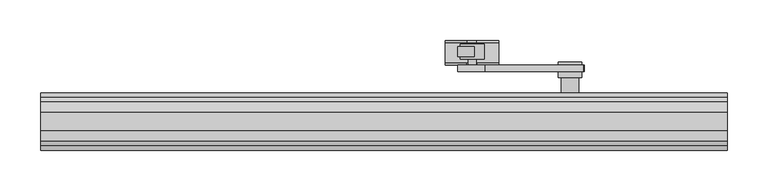
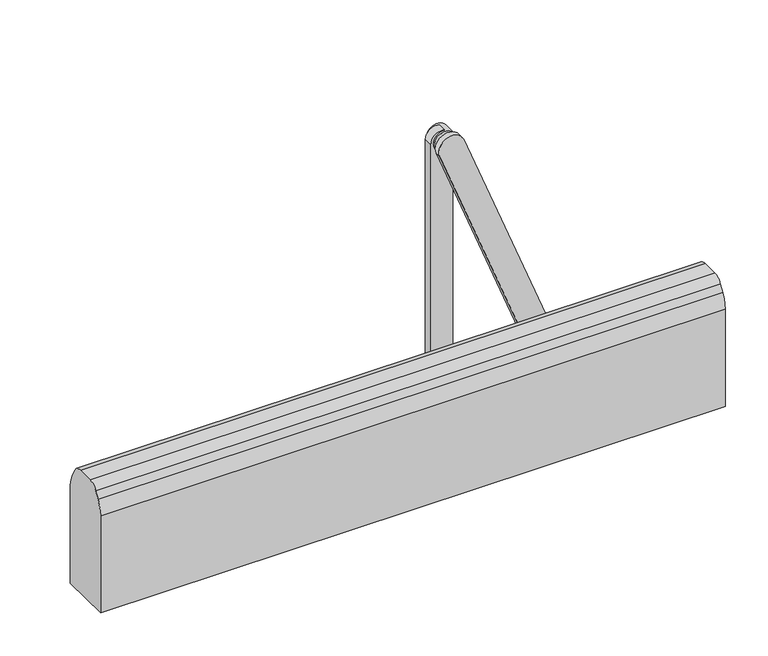
"""IFC4 building model written with IfcOpenShell, lengths in millimetres: proxy geometry, Architectural Hardware_PSW250_ASSA ABLOY_TO0261012562SI : PSW250_TO0261012562SI."""

from ifc_helpers import new_model, si_unit, point, frame, frame_2d, origin, origin_with_axes, place, context, project, spatial, polyline, circle_curve, trimmed, segment, composite_curve, outline, extrude, source, transform, mapped, element, save
from ifc_brep_helpers import plane_surface, cylinder_surface, advanced_brep


def specialty_equipment_bcced1bd(model_context):
    return source(origin(), model_context, "Body", "SolidModel", [
        advanced_brep(
        [(510.7517088, 139.6731973, 53.1484386), (540.2499715, 139.6731973, 53.1484386), (540.2499715, 139.6731973, 418.2256474), (510.7517088, 139.6731973, 418.2256474), (510.7517088, 152.1731853, 53.1484386), (510.7517088, 152.1731853, 418.2256474), (540.2465663, 152.1731853, 418.2256474), (540.2499715, 152.1731853, 53.1484386)],
        [
            (0, 1),
            (1, 2),
            (2, 3, circle_curve(frame((525.4991375, 139.6731973, 418.2256474), z_axis=(0.0, -1.0, 0.0), x_axis=(-1.0, 0.0, 0.0)), 14.7474287)),
            (3, 0),
            (4, 5),
            (5, 6, circle_curve(frame((525.4991375, 152.1731853, 418.2256474), z_axis=(0.0, 1.0, 0.0), x_axis=(-1.0, 0.0, 0.0)), 14.7474287)),
            (6, 7),
            (7, 4),
            (0, 4),
            (7, 1),
            (6, 2),
            (5, 3),
        ],
        [
            plane_surface(frame((510.7517088, 139.6731973, 53.1484386), z_axis=(0.0, -1.0, 0.0), x_axis=(0.0, 0.0, 1.0))),
            plane_surface(frame((510.7517088, 152.1731853, 53.1484386), z_axis=(0.0, 1.0, 0.0), x_axis=(0.0, 0.0, -1.0))),
            plane_surface(frame((540.2499715, 139.6731973, 53.1484386), z_axis=(0.0, 0.0, -1.0), x_axis=(0.0, 1.0, 0.0))),
            plane_surface(frame((540.2499715, 139.6731973, 418.2256474), z_axis=(1.0, 0.0, 0.0), x_axis=(0.0, 1.0, 0.0))),
            cylinder_surface(frame((525.4991375, 152.1731853, 418.2256474), z_axis=(0.0, -1.0, 0.0), x_axis=(-1.0, 0.0, 0.0)), 14.7474287),
            plane_surface(frame((510.7517088, 139.6731973, 53.1484386), z_axis=(-1.0, 0.0, 0.0), x_axis=(0.0, 1.0, 0.0))),
        ],
        [
            (0, [[1, 2, 3, 4]]),
            (1, [[5, 6, 7, 8]]),
            (2, [[9, -8, 10, -1]]),
            (3, [[-10, -7, 11, -2]]),
            (4, [[-11, -6, 12, -3]]),
            (5, [[-12, -5, -9, -4]]),
        ],
    ),
        extrude(outline(polyline([(8.0047785, 560.9664412), (38.4998129, 533.7968601), (38.4998129, 522.1399084), (8.0047785, 494.9702937), (0.0003055, 494.9702937), (0.0003055, 560.9664412), (8.0047785, 560.9664412)])), frame((0.0, 156.6731572, 0.0), z_axis=(0.0, 1.0, 0.0), x_axis=(0.0, 0.0, 1.0)), (0.0, 0.0, 1.0), 2.4999976),
        extrude(outline(polyline([(494.9702937, 129.1731834), (494.9702937, 159.1731548), (560.9664412, 159.1731548), (560.9664412, 129.1731834), (494.9702937, 129.1731834)])), origin_with_axes(), (0.0, 0.0, 1.0), 2.4999976),
        extrude(outline(composite_curve([segment(polyline([(32.3280553, 540.7175705), (53.1484386, 540.7175705), (53.1484386, 515.7846614), (32.3158361, 515.7119414)]), True, "CONTINUOUS"), segment(trimmed(circle_curve(frame_2d((24.9799343, 528.2183437)), 14.499157), [point((32.3158361, 515.7119414))], [point((32.3280553, 540.7175705))], True, "CARTESIAN"), True, "CONTINUOUS")], self_intersect=False)), frame((0.0, 141.6731715, 0.0), z_axis=(0.0, 1.0, 0.0), x_axis=(0.0, 0.0, 1.0)), (0.0, 0.0, 1.0), 4.9999952),
        extrude(outline(composite_curve([segment(trimmed(circle_curve(frame_2d((24.9799343, 528.2183437)), 14.499157), [point((24.9799343, 542.7175006))], [point((24.9799343, 513.7191867))], False, "CARTESIAN"), True, "CONTINUOUS"), segment(trimmed(circle_curve(frame_2d((24.9799343, 528.2183437)), 14.499157), [point((24.9799343, 513.7191867))], [point((24.9799343, 542.7175006))], False, "CARTESIAN"), True, "CONTINUOUS")], self_intersect=False)), frame((0.0, 136.6731763, 0.0), z_axis=(0.0, 1.0, 0.0), x_axis=(0.0, 0.0, 1.0)), (0.0, 0.0, 1.0), 14.9999857),
        extrude(outline(polyline([(8.0047785, 560.9664412), (37.5031027, 534.6848802), (37.5031027, 521.2518873), (8.0047785, 494.9702937), (-0.0192216, 494.9702937), (-0.0192216, 560.9664412), (8.0047785, 560.9664412)])), frame((0.0, 129.1731834, 0.0), z_axis=(0.0, 1.0, 0.0), x_axis=(0.0, 0.0, 1.0)), (0.0, 0.0, 1.0), 2.4999976),
        extrude(outline(composite_curve([segment(trimmed(circle_curve(frame_2d((105.4938308, 648.0113925)), 10.75), [point((105.4938308, 658.7613925))], [point((105.4938308, 637.2613925))], False, "CARTESIAN"), True, "CONTINUOUS"), segment(trimmed(circle_curve(frame_2d((105.4938308, 648.0113925)), 10.75), [point((105.4938308, 637.2613925))], [point((105.4938308, 658.7613925))], False, "CARTESIAN"), True, "CONTINUOUS")], self_intersect=False)), frame((0.0, 95.0, 0.0), z_axis=(0.0, 1.0, 0.0), x_axis=(0.0, 0.0, 1.0)), (0.0, 0.0, 1.0), 19.2731547),
        extrude(outline(composite_curve([segment(trimmed(circle_curve(frame_2d((105.4938308, 648.0113925)), 14.2491718), [point((105.4938308, 662.2605643))], [point((105.4938308, 633.7622207))], False, "CARTESIAN"), True, "CONTINUOUS"), segment(trimmed(circle_curve(frame_2d((105.4938308, 648.0113925)), 14.2491718), [point((105.4938308, 633.7622207))], [point((105.4938308, 662.2605643))], False, "CARTESIAN"), True, "CONTINUOUS")], self_intersect=False)), frame((0.0, 114.2731547, 0.0), z_axis=(0.0, 1.0, 0.0), x_axis=(0.0, 0.0, 1.0)), (0.0, 0.0, 1.0), 18.4617639),
        extrude(outline(composite_curve([segment(trimmed(circle_curve(frame_2d((418.2719569, 528.216532)), 5.0), [point((418.2719569, 533.216532))], [point((418.2719569, 523.216532))], False, "CARTESIAN"), True, "CONTINUOUS"), segment(trimmed(circle_curve(frame_2d((418.2719569, 528.216532)), 5.0), [point((418.2719569, 523.216532))], [point((418.2719569, 533.216532))], False, "CARTESIAN"), True, "CONTINUOUS")], self_intersect=False)), frame((0.0, 129.1731834, 0.0), z_axis=(0.0, 1.0, 0.0), x_axis=(0.0, 0.0, 1.0)), (0.0, 0.0, 1.0), 7.4999928),
        extrude(outline(composite_curve([segment(trimmed(circle_curve(frame_2d((418.2438317, 528.216532)), 14.5), [point((418.2438317, 542.716532))], [point((418.2438317, 513.716532))], False, "CARTESIAN"), True, "CONTINUOUS"), segment(trimmed(circle_curve(frame_2d((418.2438317, 528.216532)), 14.5), [point((418.2438317, 513.716532))], [point((418.2438317, 542.716532))], False, "CARTESIAN"), True, "CONTINUOUS")], self_intersect=False)), frame((0.0, 136.6731763, 0.0), z_axis=(0.0, 1.0, 0.0), x_axis=(0.0, 0.0, 1.0)), (0.0, 0.0, 1.0), 18.50003),
        advanced_brep(
        [(664.4157433, 121.1731672, 111.5886878), (544.2564362, 121.1731672, 425.269919), (511.878845, 121.1731672, 412.0005949), (631.7418174, 121.1731672, 99.0478304), (664.4157433, 129.1731834, 111.5886878), (631.7418174, 129.1731834, 99.0478304), (511.864313, 129.1731834, 411.9950166), (544.2564362, 129.1731834, 425.269919)],
        [
            (0, 1),
            (1, 2, circle_curve(frame((528.216532, 121.1731672, 418.2719569), z_axis=(0.0, -1.0, 0.0), x_axis=(-1.0, 0.0, 0.0)), 17.5)),
            (2, 3),
            (3, 0, circle_curve(frame((648.0113927, 121.1731672, 105.4938308), z_axis=(0.0, -1.0, 0.0), x_axis=(-1.0, 0.0, 0.0)), 17.5)),
            (4, 5, circle_curve(frame((648.0113927, 129.1731834, 105.4938308), z_axis=(0.0, 1.0, 0.0), x_axis=(-1.0, 0.0, 0.0)), 17.5)),
            (5, 6),
            (6, 7, circle_curve(frame((528.216532, 129.1731834, 418.2719569), z_axis=(0.0, 1.0, 0.0), x_axis=(-1.0, 0.0, 0.0)), 17.5)),
            (7, 4),
            (0, 4),
            (7, 1),
            (6, 2),
            (5, 3),
        ],
        [
            plane_surface(frame((630.5113927, 121.1731672, 105.4938308), z_axis=(0.0, -1.0, 0.0), x_axis=(0.0, 0.0, 1.0))),
            plane_surface(frame((630.5113927, 129.1731834, 105.4938308), z_axis=(0.0, 1.0, 0.0), x_axis=(0.0, 0.0, -1.0))),
            plane_surface(frame((544.2564362, 121.1731672, 425.269919), z_axis=(0.9338308284243376, 0.0, 0.3577149478066516), x_axis=(0.0, 1.0, 0.0))),
            cylinder_surface(frame((528.216532, 129.1731834, 418.2719569), z_axis=(0.0, -1.0, 0.0), x_axis=(-1.0, 0.0, 0.0)), 17.5),
            plane_surface(frame((631.7418174, 121.1731672, 99.0478304), z_axis=(-0.9338314444688628, 0.0, -0.3577133395907922), x_axis=(0.0, 1.0, 0.0))),
            cylinder_surface(frame((648.0113927, 129.1731834, 105.4938308), z_axis=(0.0, -1.0, 0.0), x_axis=(-1.0, 0.0, 0.0)), 17.5),
        ],
        [
            (0, [[1, 2, 3, 4]]),
            (1, [[5, 6, 7, 8]]),
            (2, [[9, -8, 10, -1]]),
            (3, [[-10, -7, 11, -2]]),
            (4, [[-11, -6, 12, -3]]),
            (5, [[-12, -5, -9, -4]]),
        ],
    ),
        advanced_brep(
        [(840.2502894, 24.9999475, 138.2889012), (840.2502894, 24.9999475, 0.0), (840.2502894, 95.0, 0.0), (840.2502894, 95.0, 138.2889012), (840.2502894, 89.647371, 158.2777994), (840.2502894, 84.3292725, 167.4958368), (840.2502894, 71.3364887, 175.0), (840.2502894, 48.6634064, 175.0), (840.2502894, 35.6706226, 167.4958368), (840.2502894, 30.3525241, 158.2777994), (0.2499715, 24.9999475, 138.2889012), (0.2499715, 30.3525241, 158.2777994), (0.2499715, 35.6706226, 167.4958368), (0.2499715, 48.6634064, 175.0), (0.2499715, 71.3364887, 175.0), (0.2499715, 84.3292725, 167.4958368), (0.2499715, 89.647371, 158.2777994), (0.2499715, 94.9999475, 138.2889012), (0.2499715, 95.0, 0.0), (0.2499715, 24.9999475, 0.0)],
        [
            (0, 1),
            (1, 2),
            (2, 3),
            (3, 4, circle_curve(frame((840.2502894, 54.9999475, 138.2889012), z_axis=(1.0, 0.0, 0.0), x_axis=(0.0, 0.0, -1.0)), 40.0)),
            (4, 5),
            (5, 6, circle_curve(frame((840.2502894, 71.3364887, 160.0), z_axis=(1.0, 0.0, 0.0), x_axis=(0.0, 0.0, -1.0)), 15.0)),
            (6, 7),
            (7, 8, circle_curve(frame((840.2502894, 48.6634064, 160.0), z_axis=(1.0, 0.0, 0.0), x_axis=(0.0, 0.0, -1.0)), 15.0)),
            (8, 9),
            (9, 0, circle_curve(frame((840.2502894, 64.9999475, 138.2889012), z_axis=(1.0, 0.0, 0.0), x_axis=(0.0, 0.0, -1.0)), 40.0)),
            (10, 11, circle_curve(frame((0.2499715, 64.9999475, 138.2889012), z_axis=(-1.0, 0.0, 0.0), x_axis=(0.0, 0.0, -1.0)), 40.0)),
            (11, 12),
            (12, 13, circle_curve(frame((0.2499715, 48.6634064, 160.0), z_axis=(-1.0, 0.0, 0.0), x_axis=(0.0, 0.0, -1.0)), 15.0)),
            (13, 14),
            (14, 15, circle_curve(frame((0.2499715, 71.3364887, 160.0), z_axis=(-1.0, 0.0, 0.0), x_axis=(0.0, 0.0, -1.0)), 15.0)),
            (15, 16),
            (16, 17, circle_curve(frame((0.2499715, 54.9999475, 138.2889012), z_axis=(-1.0, 0.0, 0.0), x_axis=(0.0, 0.0, -1.0)), 40.0)),
            (17, 18),
            (18, 19),
            (19, 10),
            (9, 11),
            (10, 0),
            (8, 12),
            (7, 13),
            (6, 14),
            (5, 15),
            (4, 16),
            (3, 17),
            (2, 18),
            (1, 19),
        ],
        [
            plane_surface(frame((840.2502894, 64.9999475, 98.2889012), z_axis=(1.0, 0.0, 0.0), x_axis=(0.0, -1.0, 0.0))),
            plane_surface(frame((0.2499715, 64.9999475, 98.2889012), z_axis=(-1.0, 0.0, 0.0), x_axis=(0.0, 1.0, 0.0))),
            cylinder_surface(frame((0.2499715, 64.9999475, 138.2889012), z_axis=(1.0, 0.0, 0.0), x_axis=(0.0, 0.0, -1.0)), 40.0),
            plane_surface(frame((840.2502894, 30.3525241, 158.2777994), z_axis=(0.0, -0.8661855860488035, 0.49972245348922545), x_axis=(-1.0, 0.0, 0.0))),
            cylinder_surface(frame((0.2499715, 48.6634064, 160.0), z_axis=(1.0, 0.0, 0.0), x_axis=(0.0, 0.0, -1.0)), 15.0),
            plane_surface(frame((840.2502894, 48.6634064, 175.0), z_axis=(0.0, 0.0, 1.0), x_axis=(-1.0, 0.0, 0.0))),
            cylinder_surface(frame((0.2499715, 71.3364887, 160.0), z_axis=(1.0, 0.0, 0.0), x_axis=(0.0, 0.0, -1.0)), 15.0),
            plane_surface(frame((840.2502894, 84.3292725, 167.4958368), z_axis=(0.0, 0.8661855860484826, 0.49972245348978145), x_axis=(-1.0, 0.0, 0.0))),
            cylinder_surface(frame((0.2499715, 54.9999475, 138.2889012), z_axis=(1.0, 0.0, 0.0), x_axis=(0.0, 0.0, -1.0)), 40.0),
            plane_surface(frame((840.2502894, 95.0, 138.2889012), z_axis=(0.0, 1.0, 0.0), x_axis=(-1.0, 0.0, 0.0))),
            plane_surface(frame((840.2502894, 95.0, 0.0), z_axis=(0.0, 0.0, -1.0), x_axis=(-1.0, 0.0, 0.0))),
            plane_surface(frame((840.2502894, 24.9999475, 0.0), z_axis=(0.0, -1.0, 0.0), x_axis=(-1.0, 0.0, 0.0))),
        ],
        [
            (0, [[1, 2, 3, 4, 5, 6, 7, 8, 9, 10]]),
            (1, [[11, 12, 13, 14, 15, 16, 17, 18, 19, 20]]),
            (2, [[21, -11, 22, -10]]),
            (3, [[23, -12, -21, -9]]),
            (4, [[24, -13, -23, -8]]),
            (5, [[25, -14, -24, -7]]),
            (6, [[26, -15, -25, -6]]),
            (7, [[27, -16, -26, -5]]),
            (8, [[28, -17, -27, -4]]),
            (9, [[29, -18, -28, -3]]),
            (10, [[30, -19, -29, -2]]),
            (11, [[-22, -20, -30, -1]]),
        ],
    ),
    ])


if __name__ == "__main__":
    model = new_model("IFC4")
    model_context = context("Model", 3, world=origin())
    ifc_project = project(units=[si_unit("LENGTHUNIT", "METRE", prefix="MILLI")], contexts=[model_context])
    site = spatial("IfcSite", under=ifc_project)
    building = spatial("IfcBuilding", under=site)
    placement = place(None, origin())
    specialty_equipment_shape = specialty_equipment_bcced1bd(model_context)
    element("IfcBuildingElementProxy", 1, Name="Architectural Hardware_PSW250_ASSA ABLOY_TO0261012562SI : PSW250_TO0261012562SI", ObjectType="Architectural Hardware_PSW250_ASSA ABLOY_TO0261012562SI : PSW250_TO0261012562SI", at=placement, inside=building, context=model_context, shape_type="MappedRepresentation", body=[
        mapped(specialty_equipment_shape, transform((0.0, 0.0, 0.0), x_axis=(1.0, 0.0, 0.0), y_axis=(0.0, 1.0, 0.0), z_axis=(0.0, 0.0, 1.0))),
    ])
    save(model, "model.ifc")

# Revit data of these elements
# Type "Architectural Hardware_PSW250_ASSA ABLOY_TO0261012562SI : PSW250_TO0261012562SI"
#   Uniclass 2.0 Description = "Door Access Controllers"
#   Uniclass 2.0 Code = "PR-25-26-xx"
#   Uniclass 1.4 Description = "Door entry token systems"
#   Uniclass 1.4 Code = "L452"
#   URL = "http://assaabloyopeningsolutions.no/prosjekt"
#   UNSPSC Code = "30171512"
#   Type Comments = "PSW250"
#   Region Europe = "NO"
#   Reference Standards = "EN 16005, EN ISO 13849-1, EN 1634-1, EN ISO 14025"
#   Provider = "ASSA ABLOY Opening Solutions Norway"
#   Product Range = "PSW250"
#   Product Guid = "bfed690d-ac7a-4c76-ae2e-3f925850da5b"
#   Product Group = "Automation Entrance Systems"
#   Product Datasheet = "http://xnet.trioving.be/Katalog.asp?ProdId=202396"
#   OmniClass Description = "Card Key Door Locking Hardware"
#   OmniClass Code = "23-17 19 11 31 11"
#   Name = "PSW250"
#   NBS Reference Description = "Door Access Controllers"
#   NBS Reference Code = "25-26-xx"
#   Model = "Architectural Hardware_PSW250_ASSA ABLOY_TO0261012562SI"
#   Manufacturer = "ASSA ABLOY"
#   ISO = "ISO 14001"
#   IFC Classification = "Door"
#   Environmental Product Declaration (EPD) = ""
#   Description = "Swing Door Operator Push"
#   Date of publishing = "2015-11-16"
#   Contact Provider = "http://assaabloyopeningsolutions.no/prosjekt"
#   BIMobject category = "Door Openers"
#   BIMobject Unique ref = "TO0261012562SI"
#   BIMobject Instructions Video = "https://www.youtube.com/user/BIMobject"
#   BIMobject Brand = "ASSA ABLOY NO"
#   Article Number = "TO0261012562SI"
#   Accessories = "Battery Backup, Elbow Switch, Safety Sensor"
#   Width [instance default] = 5' - 6.5748"
#   Offset Vertical [instance default] = 0' - 1.1811"
#   Offset Perpendicular [instance default] = 0' - 4.20333"
#   Half Width [instance default] = 2' - 9.2874"
#   Offset = 0' - 1.9685"
#   Edition number = 2
#   Finish = Silver
#   Default Elevation = 0
#   Cost = 0
# Element 1 (IfcBuildingElementProxy, "Architectural Hardware_PSW250_ASSA ABLOY_TO0261012562SI : PSW250_TO0261012562SI")
#   Offset Perpendicular = 0' - 0"
#   Materials on its faces: "Silver"
# Materials
#   "Silver": class "Metal", colour RGB 211 211 211, transparency 0, Description = "Silver", Cost = 0
